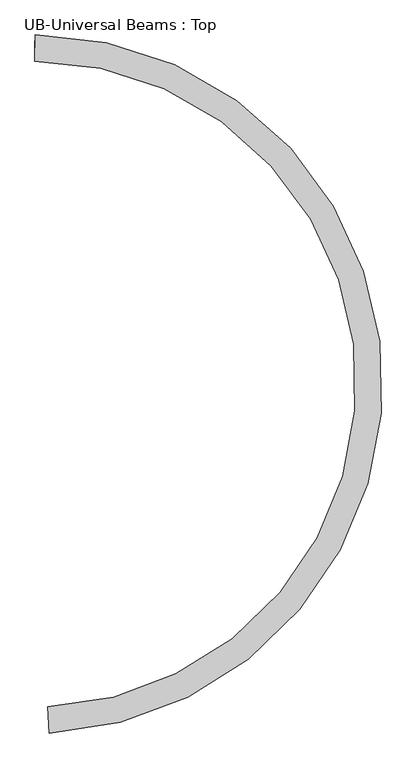
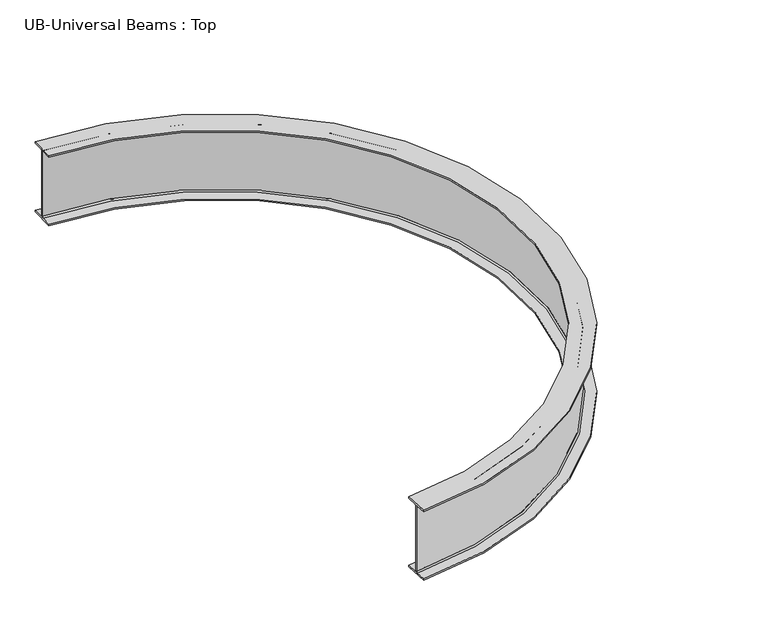
"""IFC4 building model written with IfcOpenShell, lengths in millimetres: beam geometry, UB-Universal Beams : Top."""

import ifcopenshell
import ifcopenshell.guid

model = None  # the IFC model being written
_history = None  # IfcOwnerHistory: only IFC2X3 demands one
_inside = {}  # id of a spatial element -> (the spatial element, [elements in it])
_under = {}  # id of a project, library or spatial element -> (it, [spatial elements below it])
_declared = {}  # id of a project -> (the project, [libraries it declares])
_typed = {}  # id of a type object -> (the type object, [elements of that type])
_made_of = {}  # id of a material, layer set ... -> (it, [elements and type objects made of it])


def new_model(schema):
    """Start an empty IFC model of exactly this schema.

    Asked for "IFC4X3", IfcOpenShell would pick the latest addendum, in which some entities
    have other attributes; the version numbers below select the first issue.
    IFC2X3 requires an IfcOwnerHistory on every rooted entity: one is made here for all.
    """
    global model, _history
    if schema == "IFC4X3":
        model = ifcopenshell.file(schema_version=(4, 3, 0, 0))
    else:
        model = ifcopenshell.file(schema=schema)
    _inside.clear()
    _under.clear()
    _declared.clear()
    _typed.clear()
    _made_of.clear()
    _history = None
    if model.schema == "IFC2X3":
        org = make("IfcOrganization", Name="unknown")
        user = make(
            "IfcPersonAndOrganization",
            ThePerson=make("IfcPerson", FamilyName="unknown"),
            TheOrganization=org,
        )
        app = make(
            "IfcApplication",
            ApplicationDeveloper=org,
            Version="unknown",
            ApplicationFullName="unknown",
            ApplicationIdentifier="unknown",
        )
        _history = make(
            "IfcOwnerHistory",
            OwningUser=user,
            OwningApplication=app,
            ChangeAction="ADDED",
            CreationDate=0,
        )
    return model


def make(cls, **values):
    """One entity of the class cls with the attributes given. An attribute that is None is left unset."""
    return model.create_entity(
        cls, **{name: value for name, value in values.items() if value is not None}
    )


def rooted(cls, **values):
    """An entity with a GlobalId (a new one), such as an element, a storey or a relation."""
    return make(cls, GlobalId=ifcopenshell.guid.new(), OwnerHistory=_history, **values)


def si_unit(unit_type, name, prefix=None):
    """IfcSIUnit, for example si_unit("LENGTHUNIT", "METRE", prefix="MILLI")."""
    return make("IfcSIUnit", UnitType=unit_type, Prefix=prefix, Name=name)


def assignment(units):
    """IfcUnitAssignment: the units of a project."""
    return None if units is None else make("IfcUnitAssignment", Units=units)


def point(xyz):
    """IfcCartesianPoint."""
    return None if xyz is None else make("IfcCartesianPoint", Coordinates=xyz)


def direction(xyz):
    """IfcDirection."""
    return None if xyz is None else make("IfcDirection", DirectionRatios=xyz)


def frame(location, z_axis=None, x_axis=None):
    """IfcAxis2Placement3D, a coordinate frame: its origin and axes. An axis left out is left unset."""
    return make(
        "IfcAxis2Placement3D",
        Location=point(location),
        Axis=direction(z_axis),
        RefDirection=direction(x_axis),
    )


def origin():
    """The frame at (0, 0, 0) with its axes left unset."""
    return frame((0.0, 0.0, 0.0))


def place(relative_to, where):
    """IfcLocalPlacement: puts the frame where relative to a parent placement (None: the world)."""
    return make(
        "IfcLocalPlacement", PlacementRelTo=relative_to, RelativePlacement=where
    )


def context(
    kind, dimensions, precision=None, world=None, true_north=None, identifier=None
):
    """IfcGeometricRepresentationContext, for example the 3D "Model" context."""
    return make(
        "IfcGeometricRepresentationContext",
        ContextIdentifier=identifier,
        ContextType=kind,
        CoordinateSpaceDimension=dimensions,
        Precision=precision,
        WorldCoordinateSystem=world,
        TrueNorth=true_north,
    )


def project(units=None, contexts=None):
    """IfcProject with its units and contexts."""
    return rooted(
        "IfcProject",
        Name="project",
        RepresentationContexts=contexts,
        UnitsInContext=assignment(units),
    )


def spatial(cls, under=None, at=None, **own):
    """A site, building, storey or space (cls), placed at a placement, below another one or the project."""
    s = rooted(cls, ObjectPlacement=at, **own)
    if under is not None:
        _under.setdefault(under.id(), (under, []))[1].append(s)
    return s


def polyline(points):
    """IfcPolyline through the points."""
    return make("IfcPolyline", Points=[point(p) for p in points])


def circle_curve(where, radius):
    """IfcCircle in the frame where."""
    return make("IfcCircle", Position=where, Radius=radius)


def ellipse_curve(where, semi_axis1, semi_axis2):
    """IfcEllipse in the frame where."""
    return make(
        "IfcEllipse", Position=where, SemiAxis1=semi_axis1, SemiAxis2=semi_axis2
    )


def trimmed(basis, trim1, trim2, sense, master):
    """IfcTrimmedCurve: the piece of a basis curve between two trims."""
    return make(
        "IfcTrimmedCurve",
        BasisCurve=basis,
        Trim1=trim1,
        Trim2=trim2,
        SenseAgreement=sense,
        MasterRepresentation=master,
    )


def shape(context_of_items, identifier, shape_type, items):
    """IfcShapeRepresentation: the items that make up one representation, for example the "Body"."""
    return make(
        "IfcShapeRepresentation",
        ContextOfItems=context_of_items,
        RepresentationIdentifier=identifier,
        RepresentationType=shape_type,
        Items=items,
    )


def source(mapping_origin, context_of_items, identifier, shape_type, items):
    """IfcRepresentationMap: a shape defined once, which mapped items show again and again."""
    return make(
        "IfcRepresentationMap",
        MappingOrigin=mapping_origin,
        MappedRepresentation=shape(context_of_items, identifier, shape_type, items),
    )


def transform(
    local_origin,
    x_axis=None,
    y_axis=None,
    z_axis=None,
    scale=None,
    scale2=None,
    scale3=None,
    uniform=True,
):
    """IfcCartesianTransformationOperator3D, or its non-uniform kind. x_axis, y_axis, z_axis: its Axis1, 2, 3."""
    if uniform:
        return make(
            "IfcCartesianTransformationOperator3D",
            Axis1=direction(x_axis),
            Axis2=direction(y_axis),
            LocalOrigin=point(local_origin),
            Scale=scale,
            Axis3=direction(z_axis),
        )
    return make(
        "IfcCartesianTransformationOperator3DnonUniform",
        Axis1=direction(x_axis),
        Axis2=direction(y_axis),
        LocalOrigin=point(local_origin),
        Scale=scale,
        Axis3=direction(z_axis),
        Scale2=scale2,
        Scale3=scale3,
    )


def mapped(mapping_source, mapping_target):
    """IfcMappedItem: shows the shape of a source again, moved by a transform."""
    return make(
        "IfcMappedItem", MappingSource=mapping_source, MappingTarget=mapping_target
    )


def made_of(thing, what):
    """Note that an element or type object is made of a material, layer set ...; save() writes the relation."""
    if what is not None:
        _made_of.setdefault(what.id(), (what, []))[1].append(thing)
    return thing


def element(
    cls,
    number,
    at=None,
    inside=None,
    cuts=None,
    type_object=None,
    material=None,
    context=None,
    identifier="Body",
    shape_type=None,
    held_by="IfcProductDefinitionShape",
    body=None,
    shapes=None,
    **own,
):
    """One element of the class cls, such as IfcWall. Its Tag is "e" and its number.

    at: its placement. inside: the storey or other place that contains it. cuts: it is an
    opening in that element (IfcRelVoidsElement). A single representation is given by context,
    identifier, shape_type and body (its items); several are given by shapes. held_by: the class
    of the entity that holds the representations. save() writes the other relations.
    """
    e = rooted(cls, Tag="e%d" % number, ObjectPlacement=at, **own)
    if body is not None:
        shapes = [shape(context, identifier, shape_type, body)]
    if shapes is not None:
        e.Representation = make(held_by, Representations=shapes)
    if inside is not None:
        _inside.setdefault(inside.id(), (inside, []))[1].append(e)
    if cuts is not None:
        rooted(
            "IfcRelVoidsElement", RelatingBuildingElement=cuts, RelatedOpeningElement=e
        )
    if type_object is not None:
        _typed.setdefault(type_object.id(), (type_object, []))[1].append(e)
    return made_of(e, material)


def aggregate(whole, parts):
    """IfcRelAggregates: a whole, such as a stair, and the parts it consists of."""
    return rooted("IfcRelAggregates", RelatingObject=whole, RelatedObjects=parts)


def save(model, path):
    """Write the relations noted so far, then the file.

    IfcRelAggregates (storeys below a building ...), IfcRelContainedInSpatialStructure (elements
    in a storey), IfcRelDefinesByType, IfcRelAssociatesMaterial and IfcRelDeclares: one each for
    every whole, place, type object, material and project.
    """
    for whole, parts in _under.values():
        aggregate(whole, parts)
    for where, things in _inside.values():
        rooted(
            "IfcRelContainedInSpatialStructure",
            RelatedElements=things,
            RelatingStructure=where,
        )
    for kind, things in _typed.values():
        rooted("IfcRelDefinesByType", RelatedObjects=things, RelatingType=kind)
    for what, things in _made_of.values():
        rooted("IfcRelAssociatesMaterial", RelatedObjects=things, RelatingMaterial=what)
    for by, libraries in _declared.values():
        rooted("IfcRelDeclares", RelatingContext=by, RelatedDefinitions=libraries)
    model.write(path)


def plane_surface(at):
    """IfcPlane: the flat surface through the origin of the frame at, square to its z axis."""
    return make("IfcPlane", Position=at)


def cylinder_surface(at, radius):
    """IfcCylindricalSurface: all points at the distance radius from the z axis of the frame at."""
    return make("IfcCylindricalSurface", Position=at, Radius=radius)


def revolved_surface(curve, axis_point, axis_direction):
    """IfcSurfaceOfRevolution: the curve turned about the line through axis_point along axis_direction."""
    return make(
        "IfcSurfaceOfRevolution",
        SweptCurve=make("IfcArbitraryOpenProfileDef", ProfileType="CURVE", Curve=curve),
        AxisPosition=make("IfcAxis1Placement", Location=point(axis_point), Axis=direction(axis_direction)),
    )


def advanced_brep(points, edges, surfaces, faces):
    """IfcAdvancedBrep: a solid bounded by faces that lie on surfaces and meet in shared edges.

    An edge is (start, end): straight between two places in points (the first is 0);
    or (start, end, curve); or (start, end, curve, False) where it runs against its curve.
    A face is (place in surfaces, loops), or (place, loops, False) where it looks against
    its surface's normal. A loop lists edges by number (the first is 1), with a minus sign
    where the edge is run from its end to its start. The first loop is the outer one.
    """
    corners = [point(p) for p in points]
    vertices = [make("IfcVertexPoint", VertexGeometry=c) for c in corners]
    made = []
    for start, end, *more in edges:
        made.append(
            make(
                "IfcEdgeCurve",
                EdgeStart=vertices[start],
                EdgeEnd=vertices[end],
                EdgeGeometry=more[0] if more else make("IfcPolyline", Points=[corners[start], corners[end]]),
                SameSense=more[1] if len(more) > 1 else True,
            )
        )
    hull = []
    for where, loops, *sense in faces:
        bounds = []
        for j, loop in enumerate(loops):
            ring = [make("IfcOrientedEdge", EdgeElement=made[abs(k) - 1], Orientation=k > 0) for k in loop]
            bounds.append(
                make(
                    "IfcFaceOuterBound" if j == 0 else "IfcFaceBound",
                    Bound=make("IfcEdgeLoop", EdgeList=ring),
                    Orientation=True,
                )
            )
        hull.append(make("IfcAdvancedFace", Bounds=bounds, FaceSurface=surfaces[where], SameSense=sense[0] if sense else True))
    return make("IfcAdvancedBrep", Outer=make("IfcClosedShell", CfsFaces=hull))


def ub_universal_beams_top_1b079125(model_context):
    return source(origin(), model_context, "Body", "AdvancedBrep", [
        advanced_brep(
        [(12.2060577, 4160.104149, -239.8), (12.6287274, 4230.7028838, -239.8), (12.6820102, 4239.6027243, -230.9), (12.6820102, 4239.6027243, 230.9), (12.6287274, 4230.7028838, 239.8), (12.2060577, 4160.104149, 239.8), (12.2060577, 4160.104149, 250.0), (13.1938836, 4325.101192, 250.0), (13.1938836, 4325.101192, 239.8), (12.7712138, 4254.5024573, 239.8), (12.7179311, 4245.6026168, 230.9), (12.7179311, 4245.6026168, -230.9), (12.7712138, 4254.5024573, -239.8), (13.1938836, 4325.101192, -239.8), (13.1938836, 4325.101192, -250.0), (12.2060577, 4160.104149, -250.0), (94.7315879, 84.7019896, -239.8), (94.7315879, 84.7019896, -250.0), (102.3981349, -80.1198052, -250.0), (102.3981349, -80.1198052, -239.8), (99.1177821, -9.5960554, -239.8), (98.7042532, -0.7056677, -230.9), (98.7042532, -0.7056677, 230.9), (99.1177821, -9.5960554, 239.8), (102.3981349, -80.1198052, 239.8), (102.3981349, -80.1198052, 250.0), (94.7315879, 84.7019896, 250.0), (94.7315879, 84.7019896, 239.8), (98.0119407, 14.1782398, 239.8), (98.4254696, 5.2878521, 230.9), (98.4254696, 5.2878521, -230.9), (98.0119407, 14.1782398, -239.8)],
        [
            (0, 1),
            (1, 2, circle_curve(frame((12.6287274, 4230.7028838, -230.9), z_axis=(0.999982078811149, -0.005986823576232634, 0.0), x_axis=(0.005986823576232634, 0.999982078811149, 0.0)), 8.9)),
            (2, 3),
            (3, 4, circle_curve(frame((12.6287274, 4230.7028838, 230.9), z_axis=(0.999982078811149, -0.005986823576232634, 0.0), x_axis=(0.005986823576232634, 0.999982078811149, 0.0)), 8.9)),
            (4, 5),
            (5, 6),
            (6, 7),
            (7, 8),
            (8, 9),
            (9, 10, circle_curve(frame((12.7712138, 4254.5024573, 230.9), z_axis=(0.999982078811149, -0.005986823576232634, 0.0), x_axis=(0.005986823576232634, 0.999982078811149, 0.0)), 8.9)),
            (10, 11),
            (11, 12, circle_curve(frame((12.7712138, 4254.5024573, -230.9), z_axis=(0.999982078811149, -0.005986823576232634, 0.0), x_axis=(0.005986823576232634, 0.999982078811149, 0.0)), 8.9)),
            (12, 13),
            (13, 14),
            (14, 15),
            (15, 0),
            (16, 17),
            (17, 18),
            (18, 19),
            (19, 20),
            (20, 21, circle_curve(frame((99.1177821, -9.5960554, -230.9), z_axis=(0.9989199687771112, 0.04646392125440147, 0.0), x_axis=(0.04646392125440147, -0.9989199687771112, 0.0)), 8.9)),
            (21, 22),
            (22, 23, circle_curve(frame((99.1177821, -9.5960554, 230.9), z_axis=(0.9989199687771112, 0.046463921254401463, 0.0), x_axis=(0.046463921254401463, -0.9989199687771112, 0.0)), 8.9)),
            (23, 24),
            (24, 25),
            (25, 26),
            (26, 27),
            (27, 28),
            (28, 29, circle_curve(frame((98.0119407, 14.1782398, 230.9), z_axis=(0.9989199687771112, 0.04646392125440146, 0.0), x_axis=(0.04646392125440146, -0.9989199687771112, 0.0)), 8.9)),
            (29, 30),
            (30, 31, circle_curve(frame((98.0119407, 14.1782398, -230.9), z_axis=(0.9989199687771112, 0.046463921254401463, 0.0), x_axis=(0.046463921254401463, -0.9989199687771112, 0.0)), 8.9)),
            (31, 16),
            (0, 16, circle_curve(frame((0.0, 2121.3203436, -239.8), z_axis=(0.0, 0.0, -1.0), x_axis=(0.0, -1.0, 0.0)), 2038.8203436)),
            (31, 1, circle_curve(frame((0.0, 2121.3203436, -239.8), z_axis=(0.0, 0.0, 1.0), x_axis=(0.0, -1.0, 0.0)), 2109.4203436)),
            (30, 2, circle_curve(frame((0.0, 2121.3203436, -230.9), z_axis=(0.0, 0.0, 1.0), x_axis=(0.0, -1.0, 0.0)), 2118.3203436)),
            (29, 3, circle_curve(frame((0.0, 2121.3203436, 230.9), z_axis=(0.0, 0.0, 1.0), x_axis=(0.0, -1.0, 0.0)), 2118.3203436)),
            (28, 4, circle_curve(frame((0.0, 2121.3203436, 239.8), z_axis=(0.0, 0.0, 1.0), x_axis=(0.0, -1.0, 0.0)), 2109.4203436)),
            (27, 5, circle_curve(frame((0.0, 2121.3203436, 239.8), z_axis=(0.0, 0.0, 1.0), x_axis=(0.0, -1.0, 0.0)), 2038.8203436)),
            (26, 6, circle_curve(frame((0.0, 2121.3203436, 250.0), z_axis=(0.0, 0.0, 1.0), x_axis=(0.0, -1.0, 0.0)), 2038.8203436)),
            (25, 7, circle_curve(frame((0.0, 2121.3203436, 250.0), z_axis=(0.0, 0.0, 1.0), x_axis=(0.0, -1.0, 0.0)), 2203.8203436)),
            (24, 8, circle_curve(frame((0.0, 2121.3203436, 239.8), z_axis=(0.0, 0.0, 1.0), x_axis=(0.0, -1.0, 0.0)), 2203.8203436)),
            (23, 9, circle_curve(frame((0.0, 2121.3203436, 239.8), z_axis=(0.0, 0.0, 1.0), x_axis=(0.0, -1.0, 0.0)), 2133.2203436)),
            (22, 10, circle_curve(frame((0.0, 2121.3203436, 230.9), z_axis=(0.0, 0.0, 1.0), x_axis=(0.0, -1.0, 0.0)), 2124.3203436)),
            (21, 11, circle_curve(frame((0.0, 2121.3203436, -230.9), z_axis=(0.0, 0.0, 1.0), x_axis=(0.0, -1.0, 0.0)), 2124.3203436)),
            (20, 12, circle_curve(frame((0.0, 2121.3203436, -239.8), z_axis=(0.0, 0.0, 1.0), x_axis=(0.0, -1.0, 0.0)), 2133.2203436)),
            (19, 13, circle_curve(frame((0.0, 2121.3203436, -239.8), z_axis=(0.0, 0.0, 1.0), x_axis=(0.0, -1.0, 0.0)), 2203.8203436)),
            (18, 14, circle_curve(frame((0.0, 2121.3203436, -250.0), z_axis=(0.0, 0.0, 1.0), x_axis=(0.0, -1.0, 0.0)), 2203.8203436)),
            (17, 15, circle_curve(frame((0.0, 2121.3203436, -250.0), z_axis=(0.0, 0.0, 1.0), x_axis=(0.0, -1.0, 0.0)), 2038.8203436)),
        ],
        [
            plane_surface(frame((12.6999706, 4242.6026705, 0.0), z_axis=(-0.9999820788111491, 0.005986823576233079, 0.0), x_axis=(0.0, 0.0, 1.0))),
            plane_surface(frame((98.5648614, 2.2910922, 0.0), z_axis=(-0.9989199687771112, -0.046463921254401394, 0.0), x_axis=(0.0, 0.0, 1.0))),
            plane_surface(frame((0.0, 2121.3203436, -239.8), z_axis=(0.0, 0.0, 1.0), x_axis=(0.0, -1.0, 0.0))),
            revolved_surface(trimmed(ellipse_curve(frame((0.0, 11.9, -230.9), z_axis=(1.0, 0.0, 0.0), x_axis=(0.0, -1.0, 0.0)), 8.9, 8.9), [point((0.0, 3.0, -230.9))], [point((0.0, 11.9, -239.8))], True, "CARTESIAN"), (0.0, 2121.3203436, 0.0), (0.0, 0.0, 1.0)),
            revolved_surface(polyline([(0.0, 3.0, 230.9), (0.0, 3.0, -230.9)]), (0.0, 2121.3203436, 0.0), (0.0, 0.0, 1.0)),
            revolved_surface(trimmed(ellipse_curve(frame((0.0, 11.9, 230.9), z_axis=(1.0, 0.0, 0.0), x_axis=(0.0, -1.0, 0.0)), 8.9, 8.9), [point((0.0, 11.9, 239.8))], [point((0.0, 3.0, 230.9))], True, "CARTESIAN"), (0.0, 2121.3203436, 0.0), (0.0, 0.0, 1.0)),
            plane_surface(frame((0.0, 2121.3203436, 239.8), z_axis=(0.0, 0.0, -1.0), x_axis=(0.0, -1.0, 0.0))),
            revolved_surface(polyline([(0.0, 82.5, 250.0), (0.0, 82.5, 239.8)]), (0.0, 2121.3203436, 0.0), (0.0, 0.0, 1.0)),
            plane_surface(frame((0.0, 2121.3203436, 250.0), z_axis=(0.0, 0.0, 1.0), x_axis=(0.0, -1.0, 0.0))),
            cylinder_surface(frame((0.0, 2121.3203436, 0.0), z_axis=(0.0, 0.0, 1.0), x_axis=(0.0, -1.0, 0.0)), 2203.8203436),
            revolved_surface(trimmed(ellipse_curve(frame((0.0, -11.9, 230.9), z_axis=(1.0, 0.0, 0.0), x_axis=(0.0, -1.0, 0.0)), 8.9, 8.9), [point((0.0, -3.0, 230.9))], [point((0.0, -11.9, 239.8))], True, "CARTESIAN"), (0.0, 2121.3203436, 0.0), (0.0, 0.0, 1.0)),
            cylinder_surface(frame((0.0, 2121.3203436, 0.0), z_axis=(0.0, 0.0, 1.0), x_axis=(0.0, -1.0, 0.0)), 2124.3203436),
            revolved_surface(trimmed(ellipse_curve(frame((0.0, -11.9, -230.9), z_axis=(1.0, 0.0, 0.0), x_axis=(0.0, -1.0, 0.0)), 8.9, 8.9), [point((0.0, -11.9, -239.8))], [point((0.0, -3.0, -230.9))], True, "CARTESIAN"), (0.0, 2121.3203436, 0.0), (0.0, 0.0, 1.0)),
            plane_surface(frame((0.0, 2121.3203436, -250.0), z_axis=(0.0, 0.0, -1.0), x_axis=(0.0, -1.0, 0.0))),
            revolved_surface(polyline([(0.0, 82.5, -239.8), (0.0, 82.5, -250.0)]), (0.0, 2121.3203436, 0.0), (0.0, 0.0, 1.0)),
        ],
        [
            (0, [[1, 2, 3, 4, 5, 6, 7, 8, 9, 10, 11, 12, 13, 14, 15, 16]]),
            (1, [[17, 18, 19, 20, 21, 22, 23, 24, 25, 26, 27, 28, 29, 30, 31, 32]]),
            (2, [[-1, 33, -32, 34]]),
            (3, [[-2, -34, -31, 35]]),
            (4, [[-3, -35, -30, 36]]),
            (5, [[-4, -36, -29, 37]]),
            (6, [[-5, -37, -28, 38]]),
            (7, [[-6, -38, -27, 39]]),
            (8, [[-7, -39, -26, 40]]),
            (9, [[-8, -40, -25, 41]]),
            (6, [[-9, -41, -24, 42]]),
            (10, [[-10, -42, -23, 43]]),
            (11, [[-11, -43, -22, 44]]),
            (12, [[-12, -44, -21, 45]]),
            (2, [[-13, -45, -20, 46]]),
            (9, [[-14, -46, -19, 47]]),
            (13, [[-15, -47, -18, 48]]),
            (14, [[-16, -48, -17, -33]]),
        ],
    ),
    ])


if __name__ == "__main__":
    model = new_model("IFC4")
    model_context = context("Model", 3, world=origin())
    ifc_project = project(units=[si_unit("LENGTHUNIT", "METRE", prefix="MILLI")], contexts=[model_context])
    site = spatial("IfcSite", under=ifc_project)
    building = spatial("IfcBuilding", under=site)
    placement = place(None, origin())
    ub_universal_beams_top_shape = ub_universal_beams_top_1b079125(model_context)
    element("IfcBeam", 1, ObjectType="UB-Universal Beams : Top", at=placement, inside=building, context=model_context, shape_type="MappedRepresentation", body=[
        mapped(ub_universal_beams_top_shape, transform((0.0, 0.0, 0.0), x_axis=(1.0, 0.0, 0.0), y_axis=(0.0, 1.0, 0.0), z_axis=(0.0, 0.0, 1.0))),
    ])
    save(model, "model.ifc")

# Revit data of these elements
# Type "UB-Universal Beams : Top"
#   Section Name Key = "UB305X165X40"
#   Width = 165 mm
#   Web Thickness = 6 mm
#   Web Fillet = 8.9 mm
#   Warping Constant = 164000 cm⁶
#   Torsional Moment of Inertia = 14.7 cm⁴
#   Section Area = 51.3 cm²
#   Plastic Modulus weak axis = 0.00501468 (stored number, unit not read)
#   Plastic Modulus strong axis = 0.022001 (stored number, unit not read)
#   Nominal Weight = 395.207 N/m
#   Moment of Inertia weak axis = 764 cm⁴
#   Moment of Inertia strong axis = 8503 cm⁴
#   Height = 500 mm
#   Flange Thickness = 10.2 mm
#   Elastic Modulus weak axis = 0.00327014 (stored number, unit not read)
#   Elastic Modulus strong axis = 0.0197762 (stored number, unit not read)
#   Centroid Vertical = 250 mm
#   Centroid Horizontal = 82.5 mm
#   Length [instance default] = 1500 mm
#   Structural Material [instance default] = Metal - Steel 43-275
#   Type Comments = ""
#   Assembly Code = ""
# Element 1 (IfcBeam, "UB-Universal Beams : Top")
#   Materials on its faces: "Metal - Steel 43-275"
# Materials
#   "Metal - Steel 43-275": class "Metal", colour RGB 247 247 247, transparency 0, Cost = 0
